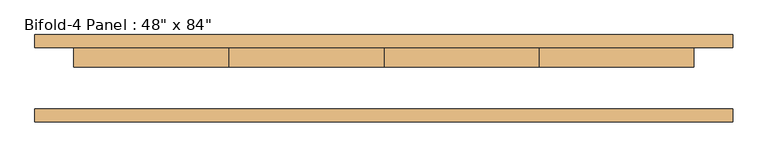
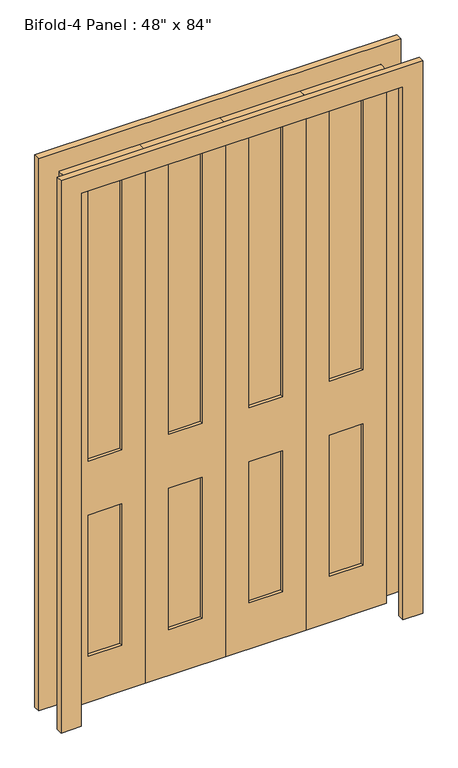
"""IFC4 building model written with IfcOpenShell, lengths in millimetres: door geometry."""

from ifc_helpers import new_model, si_unit, frame, origin, place, context, project, spatial, polyline, outline, extrude, source, transform, mapped, element, save


def door_e6393cd6(model_context):
    return source(origin(), model_context, "Body", "SweptSolid", [
        extrude(outline(polyline([(393.7, 47.625), (520.7, 47.625), (520.7, 34.925), (393.7, 34.925), (393.7, 47.625)])), frame((0.0, 0.0, 965.2), z_axis=(0.0, 0.0, 1.0), x_axis=(1.0, 0.0, 0.0)), (0.0, 0.0, 1.0), 1085.85),
        extrude(outline(polyline([(393.7, 47.625), (520.7, 47.625), (520.7, 34.925), (393.7, 34.925), (393.7, 47.625)])), frame((0.0, 0.0, 184.15), z_axis=(0.0, 0.0, 1.0), x_axis=(1.0, 0.0, 0.0)), (0.0, 0.0, 1.0), 565.15),
        extrude(outline(polyline([(88.9, 47.625), (215.9, 47.625), (215.9, 34.925), (88.9, 34.925), (88.9, 47.625)])), frame((0.0, 0.0, 965.2), z_axis=(0.0, 0.0, 1.0), x_axis=(1.0, 0.0, 0.0)), (0.0, 0.0, 1.0), 1085.85),
        extrude(outline(polyline([(88.9, 47.625), (215.9, 47.625), (215.9, 34.925), (88.9, 34.925), (88.9, 47.625)])), frame((0.0, 0.0, 184.15), z_axis=(0.0, 0.0, 1.0), x_axis=(1.0, 0.0, 0.0)), (0.0, 0.0, 1.0), 565.15),
        extrude(outline(polyline([(-215.9, 47.625), (-88.9, 47.625), (-88.9, 34.925), (-215.9, 34.925), (-215.9, 47.625)])), frame((0.0, 0.0, 184.15), z_axis=(0.0, 0.0, 1.0), x_axis=(1.0, 0.0, 0.0)), (0.0, 0.0, 1.0), 565.15),
        extrude(outline(polyline([(-215.9, 47.625), (-88.9, 47.625), (-88.9, 34.925), (-215.9, 34.925), (-215.9, 47.625)])), frame((0.0, 0.0, 965.2), z_axis=(0.0, 0.0, 1.0), x_axis=(1.0, 0.0, 0.0)), (0.0, 0.0, 1.0), 1085.85),
        extrude(outline(polyline([(-520.7, 47.625), (-393.7, 47.625), (-393.7, 34.925), (-520.7, 34.925), (-520.7, 47.625)])), frame((0.0, 0.0, 965.2), z_axis=(0.0, 0.0, 1.0), x_axis=(1.0, 0.0, 0.0)), (0.0, 0.0, 1.0), 1085.85),
        extrude(outline(polyline([(-520.7, 47.625), (-393.7, 47.625), (-393.7, 34.925), (-520.7, 34.925), (-520.7, 47.625)])), frame((0.0, 0.0, 184.15), z_axis=(0.0, 0.0, 1.0), x_axis=(1.0, 0.0, 0.0)), (0.0, 0.0, 1.0), 565.15),
        extrude(outline(polyline([(0.0, 685.8), (2209.8, 685.8), (2209.8, -685.8), (0.0, -685.8), (0.0, -609.6), (2133.6, -609.6), (2133.6, 609.6), (0.0, 609.6), (0.0, 685.8)])), frame((0.0, -85.725, 0.0), z_axis=(0.0, 1.0, 0.0), x_axis=(0.0, 0.0, 1.0)), (0.0, 0.0, 1.0), 25.4),
        extrude(outline(polyline([(0.0, 685.8), (2209.8, 685.8), (2209.8, -685.8), (0.0, -685.8), (0.0, -609.6), (2133.6, -609.6), (2133.6, 609.6), (0.0, 609.6), (0.0, 685.8)])), frame((0.0, 60.325, 0.0), z_axis=(0.0, 1.0, 0.0), x_axis=(0.0, 0.0, 1.0)), (0.0, 0.0, 1.0), 25.4),
        extrude(outline(polyline([(0.0, -609.6), (0.0, -304.8), (2133.6, -304.8), (2133.6, -609.6), (0.0, -609.6)]), holes=[polyline([(2051.05, -520.7), (2051.05, -393.7), (965.2, -393.7), (965.2, -520.7), (2051.05, -520.7)]), polyline([(749.3, -520.7), (749.3, -393.7), (184.15, -393.7), (184.15, -520.7), (749.3, -520.7)])]), frame((0.0, 22.225, 0.0), z_axis=(0.0, 1.0, 0.0), x_axis=(0.0, 0.0, 1.0)), (0.0, 0.0, 1.0), 38.1),
        extrude(outline(polyline([(0.0, -304.8), (0.0, 0.0), (2133.6, 0.0), (2133.6, -304.8), (0.0, -304.8)]), holes=[polyline([(2051.05, -215.9), (2051.05, -88.9), (965.2, -88.9), (965.2, -215.9), (2051.05, -215.9)]), polyline([(749.3, -215.9), (749.3, -88.9), (184.15, -88.9), (184.15, -215.9), (749.3, -215.9)])]), frame((0.0, 22.225, 0.0), z_axis=(0.0, 1.0, 0.0), x_axis=(0.0, 0.0, 1.0)), (0.0, 0.0, 1.0), 38.1),
        extrude(outline(polyline([(0.0, 0.0), (0.0, 304.8), (2133.6, 304.8), (2133.6, 0.0), (0.0, 0.0)]), holes=[polyline([(2051.05, 88.9), (2051.05, 215.9), (965.2, 215.9), (965.2, 88.9), (2051.05, 88.9)]), polyline([(749.3, 88.9), (749.3, 215.9), (184.15, 215.9), (184.15, 88.9), (749.3, 88.9)])]), frame((0.0, 22.225, 0.0), z_axis=(0.0, 1.0, 0.0), x_axis=(0.0, 0.0, 1.0)), (0.0, 0.0, 1.0), 38.1),
        extrude(outline(polyline([(0.0, 304.8), (0.0, 609.6), (2133.6, 609.6), (2133.6, 304.8), (0.0, 304.8)]), holes=[polyline([(2051.05, 393.7), (2051.05, 520.7), (965.2, 520.7), (965.2, 393.7), (2051.05, 393.7)]), polyline([(749.3, 393.7), (749.3, 520.7), (184.15, 520.7), (184.15, 393.7), (749.3, 393.7)])]), frame((0.0, 22.225, 0.0), z_axis=(0.0, 1.0, 0.0), x_axis=(0.0, 0.0, 1.0)), (0.0, 0.0, 1.0), 38.1),
    ])


if __name__ == "__main__":
    model = new_model("IFC4")
    model_context = context("Model", 3, world=origin())
    ifc_project = project(units=[si_unit("LENGTHUNIT", "METRE", prefix="MILLI")], contexts=[model_context])
    site = spatial("IfcSite", under=ifc_project)
    building = spatial("IfcBuilding", under=site)
    placement = place(None, origin())
    door_shape = door_e6393cd6(model_context)
    element("IfcDoor", 1, ObjectType="Bifold-4 Panel : 48\" x 84\"", at=placement, inside=building, context=model_context, shape_type="MappedRepresentation", body=[
        mapped(door_shape, transform((0.0, 0.0, 0.0), x_axis=(1.0, 0.0, 0.0), y_axis=(0.0, 1.0, 0.0), z_axis=(0.0, 0.0, 1.0))),
    ])
    save(model, "model.ifc")

# Revit data of these elements
# Type "Bifold-4 Panel : 48\" x 84\""
#   Type Mark = "38"
#   Assembly Code = "C1020"
#   Thickness = 0' - 1 1/2"
#   Height = 7' - 0"
#   Trim Width = 0' - 3"
#   Width = 4' - 0"
#   Door Material = Door - Panel
#   Frame Material = Door - Frame
#   Function = (empty or 0)
#   Description = (empty or 0)
#   Wall Closure = (empty or 0)
# Element 1 (IfcDoor, "Bifold-4 Panel : 48\" x 84\"")
#   Materials on its faces: "Door - Panel", "Door - Frame"
# Materials
#   "Door - Panel": class "Wood", colour RGB 210 159 95, transparency 0, Cost = 0
#   "Door - Frame": class "Miscellaneous", colour RGB 118 70 51, transparency 0, Cost = 0
